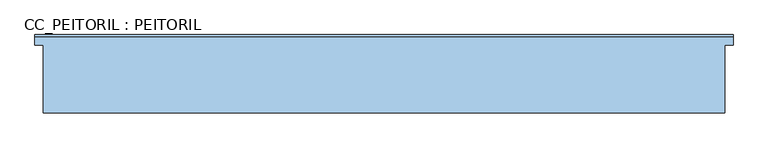
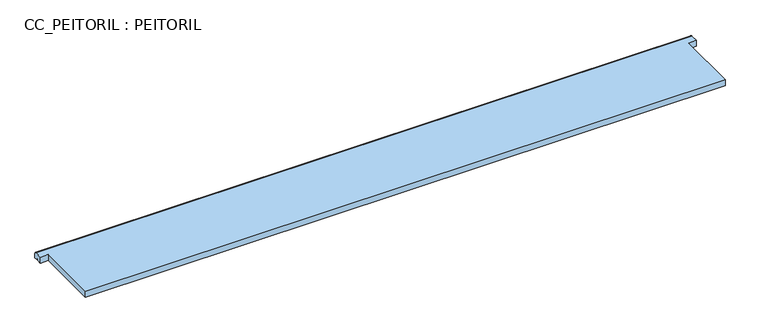
"""IFC4 building model written with IfcOpenShell, lengths in millimetres: window geometry, CC_PEITORIL : PEITORIL."""

import ifcopenshell
import ifcopenshell.guid

model = None  # the IFC model being written
_history = None  # IfcOwnerHistory: only IFC2X3 demands one
_inside = {}  # id of a spatial element -> (the spatial element, [elements in it])
_under = {}  # id of a project, library or spatial element -> (it, [spatial elements below it])
_declared = {}  # id of a project -> (the project, [libraries it declares])
_typed = {}  # id of a type object -> (the type object, [elements of that type])
_made_of = {}  # id of a material, layer set ... -> (it, [elements and type objects made of it])


def new_model(schema):
    """Start an empty IFC model of exactly this schema.

    Asked for "IFC4X3", IfcOpenShell would pick the latest addendum, in which some entities
    have other attributes; the version numbers below select the first issue.
    IFC2X3 requires an IfcOwnerHistory on every rooted entity: one is made here for all.
    """
    global model, _history
    if schema == "IFC4X3":
        model = ifcopenshell.file(schema_version=(4, 3, 0, 0))
    else:
        model = ifcopenshell.file(schema=schema)
    _inside.clear()
    _under.clear()
    _declared.clear()
    _typed.clear()
    _made_of.clear()
    _history = None
    if model.schema == "IFC2X3":
        org = make("IfcOrganization", Name="unknown")
        user = make(
            "IfcPersonAndOrganization",
            ThePerson=make("IfcPerson", FamilyName="unknown"),
            TheOrganization=org,
        )
        app = make(
            "IfcApplication",
            ApplicationDeveloper=org,
            Version="unknown",
            ApplicationFullName="unknown",
            ApplicationIdentifier="unknown",
        )
        _history = make(
            "IfcOwnerHistory",
            OwningUser=user,
            OwningApplication=app,
            ChangeAction="ADDED",
            CreationDate=0,
        )
    return model


def make(cls, **values):
    """One entity of the class cls with the attributes given. An attribute that is None is left unset."""
    return model.create_entity(
        cls, **{name: value for name, value in values.items() if value is not None}
    )


def rooted(cls, **values):
    """An entity with a GlobalId (a new one), such as an element, a storey or a relation."""
    return make(cls, GlobalId=ifcopenshell.guid.new(), OwnerHistory=_history, **values)


def si_unit(unit_type, name, prefix=None):
    """IfcSIUnit, for example si_unit("LENGTHUNIT", "METRE", prefix="MILLI")."""
    return make("IfcSIUnit", UnitType=unit_type, Prefix=prefix, Name=name)


def assignment(units):
    """IfcUnitAssignment: the units of a project."""
    return None if units is None else make("IfcUnitAssignment", Units=units)


def point(xyz):
    """IfcCartesianPoint."""
    return None if xyz is None else make("IfcCartesianPoint", Coordinates=xyz)


def direction(xyz):
    """IfcDirection."""
    return None if xyz is None else make("IfcDirection", DirectionRatios=xyz)


def frame(location, z_axis=None, x_axis=None):
    """IfcAxis2Placement3D, a coordinate frame: its origin and axes. An axis left out is left unset."""
    return make(
        "IfcAxis2Placement3D",
        Location=point(location),
        Axis=direction(z_axis),
        RefDirection=direction(x_axis),
    )


def origin():
    """The frame at (0, 0, 0) with its axes left unset."""
    return frame((0.0, 0.0, 0.0))


def place(relative_to, where):
    """IfcLocalPlacement: puts the frame where relative to a parent placement (None: the world)."""
    return make(
        "IfcLocalPlacement", PlacementRelTo=relative_to, RelativePlacement=where
    )


def context(
    kind, dimensions, precision=None, world=None, true_north=None, identifier=None
):
    """IfcGeometricRepresentationContext, for example the 3D "Model" context."""
    return make(
        "IfcGeometricRepresentationContext",
        ContextIdentifier=identifier,
        ContextType=kind,
        CoordinateSpaceDimension=dimensions,
        Precision=precision,
        WorldCoordinateSystem=world,
        TrueNorth=true_north,
    )


def project(units=None, contexts=None):
    """IfcProject with its units and contexts."""
    return rooted(
        "IfcProject",
        Name="project",
        RepresentationContexts=contexts,
        UnitsInContext=assignment(units),
    )


def spatial(cls, under=None, at=None, **own):
    """A site, building, storey or space (cls), placed at a placement, below another one or the project."""
    s = rooted(cls, ObjectPlacement=at, **own)
    if under is not None:
        _under.setdefault(under.id(), (under, []))[1].append(s)
    return s


def circle_curve(where, radius):
    """IfcCircle in the frame where."""
    return make("IfcCircle", Position=where, Radius=radius)


def shape(context_of_items, identifier, shape_type, items):
    """IfcShapeRepresentation: the items that make up one representation, for example the "Body"."""
    return make(
        "IfcShapeRepresentation",
        ContextOfItems=context_of_items,
        RepresentationIdentifier=identifier,
        RepresentationType=shape_type,
        Items=items,
    )


def source(mapping_origin, context_of_items, identifier, shape_type, items):
    """IfcRepresentationMap: a shape defined once, which mapped items show again and again."""
    return make(
        "IfcRepresentationMap",
        MappingOrigin=mapping_origin,
        MappedRepresentation=shape(context_of_items, identifier, shape_type, items),
    )


def transform(
    local_origin,
    x_axis=None,
    y_axis=None,
    z_axis=None,
    scale=None,
    scale2=None,
    scale3=None,
    uniform=True,
):
    """IfcCartesianTransformationOperator3D, or its non-uniform kind. x_axis, y_axis, z_axis: its Axis1, 2, 3."""
    if uniform:
        return make(
            "IfcCartesianTransformationOperator3D",
            Axis1=direction(x_axis),
            Axis2=direction(y_axis),
            LocalOrigin=point(local_origin),
            Scale=scale,
            Axis3=direction(z_axis),
        )
    return make(
        "IfcCartesianTransformationOperator3DnonUniform",
        Axis1=direction(x_axis),
        Axis2=direction(y_axis),
        LocalOrigin=point(local_origin),
        Scale=scale,
        Axis3=direction(z_axis),
        Scale2=scale2,
        Scale3=scale3,
    )


def mapped(mapping_source, mapping_target):
    """IfcMappedItem: shows the shape of a source again, moved by a transform."""
    return make(
        "IfcMappedItem", MappingSource=mapping_source, MappingTarget=mapping_target
    )


def made_of(thing, what):
    """Note that an element or type object is made of a material, layer set ...; save() writes the relation."""
    if what is not None:
        _made_of.setdefault(what.id(), (what, []))[1].append(thing)
    return thing


def element(
    cls,
    number,
    at=None,
    inside=None,
    cuts=None,
    type_object=None,
    material=None,
    context=None,
    identifier="Body",
    shape_type=None,
    held_by="IfcProductDefinitionShape",
    body=None,
    shapes=None,
    **own,
):
    """One element of the class cls, such as IfcWall. Its Tag is "e" and its number.

    at: its placement. inside: the storey or other place that contains it. cuts: it is an
    opening in that element (IfcRelVoidsElement). A single representation is given by context,
    identifier, shape_type and body (its items); several are given by shapes. held_by: the class
    of the entity that holds the representations. save() writes the other relations.
    """
    e = rooted(cls, Tag="e%d" % number, ObjectPlacement=at, **own)
    if body is not None:
        shapes = [shape(context, identifier, shape_type, body)]
    if shapes is not None:
        e.Representation = make(held_by, Representations=shapes)
    if inside is not None:
        _inside.setdefault(inside.id(), (inside, []))[1].append(e)
    if cuts is not None:
        rooted(
            "IfcRelVoidsElement", RelatingBuildingElement=cuts, RelatedOpeningElement=e
        )
    if type_object is not None:
        _typed.setdefault(type_object.id(), (type_object, []))[1].append(e)
    return made_of(e, material)


def aggregate(whole, parts):
    """IfcRelAggregates: a whole, such as a stair, and the parts it consists of."""
    return rooted("IfcRelAggregates", RelatingObject=whole, RelatedObjects=parts)


def save(model, path):
    """Write the relations noted so far, then the file.

    IfcRelAggregates (storeys below a building ...), IfcRelContainedInSpatialStructure (elements
    in a storey), IfcRelDefinesByType, IfcRelAssociatesMaterial and IfcRelDeclares: one each for
    every whole, place, type object, material and project.
    """
    for whole, parts in _under.values():
        aggregate(whole, parts)
    for where, things in _inside.values():
        rooted(
            "IfcRelContainedInSpatialStructure",
            RelatedElements=things,
            RelatingStructure=where,
        )
    for kind, things in _typed.values():
        rooted("IfcRelDefinesByType", RelatedObjects=things, RelatingType=kind)
    for what, things in _made_of.values():
        rooted("IfcRelAssociatesMaterial", RelatedObjects=things, RelatingMaterial=what)
    for by, libraries in _declared.values():
        rooted("IfcRelDeclares", RelatingContext=by, RelatedDefinitions=libraries)
    model.write(path)


def plane_surface(at):
    """IfcPlane: the flat surface through the origin of the frame at, square to its z axis."""
    return make("IfcPlane", Position=at)


def cylinder_surface(at, radius):
    """IfcCylindricalSurface: all points at the distance radius from the z axis of the frame at."""
    return make("IfcCylindricalSurface", Position=at, Radius=radius)


def advanced_brep(points, edges, surfaces, faces):
    """IfcAdvancedBrep: a solid bounded by faces that lie on surfaces and meet in shared edges.

    An edge is (start, end): straight between two places in points (the first is 0);
    or (start, end, curve); or (start, end, curve, False) where it runs against its curve.
    A face is (place in surfaces, loops), or (place, loops, False) where it looks against
    its surface's normal. A loop lists edges by number (the first is 1), with a minus sign
    where the edge is run from its end to its start. The first loop is the outer one.
    """
    corners = [point(p) for p in points]
    vertices = [make("IfcVertexPoint", VertexGeometry=c) for c in corners]
    made = []
    for start, end, *more in edges:
        made.append(
            make(
                "IfcEdgeCurve",
                EdgeStart=vertices[start],
                EdgeEnd=vertices[end],
                EdgeGeometry=more[0] if more else make("IfcPolyline", Points=[corners[start], corners[end]]),
                SameSense=more[1] if len(more) > 1 else True,
            )
        )
    hull = []
    for where, loops, *sense in faces:
        bounds = []
        for j, loop in enumerate(loops):
            ring = [make("IfcOrientedEdge", EdgeElement=made[abs(k) - 1], Orientation=k > 0) for k in loop]
            bounds.append(
                make(
                    "IfcFaceOuterBound" if j == 0 else "IfcFaceBound",
                    Bound=make("IfcEdgeLoop", EdgeList=ring),
                    Orientation=True,
                )
            )
        hull.append(make("IfcAdvancedFace", Bounds=bounds, FaceSurface=surfaces[where], SameSense=sense[0] if sense else True))
    return make("IfcAdvancedBrep", Outer=make("IfcClosedShell", CfsFaces=hull))


def cc_peitoril_peitoril_3c142dd7(model_context):
    return source(origin(), model_context, "Body", "AdvancedBrep", [
        advanced_brep(
        [(-1000.0, 100.0, 1500.0), (-1000.0, -100.0, 1500.0), (1000.0, -100.0, 1500.0), (1000.0, 100.0, 1500.0), (1025.0, 100.0, 1500.0), (1025.0, 123.4916648, 1500.0), (-1025.0, 123.4916648, 1500.0), (-1025.0, 100.0, 1500.0), (-1000.0, 100.0, 1480.0), (-1025.0, 100.0, 1480.0), (-1025.0, 115.0, 1480.0), (1025.0, 115.0, 1480.0), (1025.0, 100.0, 1480.0), (1000.0, 100.0, 1480.0), (1000.0, -100.0, 1480.0), (-1000.0, -100.0, 1480.0), (-1025.0, 130.0, 1480.0), (1025.0, 130.0, 1480.0), (1025.0, 120.0, 1480.0), (-1025.0, 120.0, 1480.0), (1025.0, 115.0, 1485.0), (1025.0, 120.0, 1485.0), (1025.0, 130.0, 1493.4916648), (-1025.0, 130.0, 1493.4916648), (-1025.0, 120.0, 1485.0), (-1025.0, 115.0, 1485.0)],
        [
            (0, 1),
            (1, 2),
            (2, 3),
            (3, 4),
            (4, 5),
            (5, 6),
            (6, 7),
            (7, 0),
            (8, 9),
            (9, 10),
            (10, 11),
            (11, 12),
            (12, 13),
            (13, 14),
            (14, 15),
            (15, 8),
            (16, 17),
            (17, 18),
            (18, 19),
            (19, 16),
            (0, 8),
            (15, 1),
            (14, 2),
            (13, 3),
            (12, 4),
            (11, 20),
            (20, 21),
            (21, 18),
            (17, 22),
            (22, 5, circle_curve(frame((1025.0, 123.4916648, 1493.4916648), z_axis=(1.0, 0.0, 0.0), x_axis=(0.0, -1.0, 0.0)), 6.5083352)),
            (16, 23),
            (23, 22),
            (9, 7),
            (6, 23, circle_curve(frame((-1025.0, 123.4916648, 1493.4916648), z_axis=(-1.0, 0.0, 0.0), x_axis=(0.0, -1.0, 0.0)), 6.5083352)),
            (19, 24),
            (24, 25),
            (25, 10),
            (24, 21),
            (20, 25),
        ],
        [
            plane_surface(frame((-1000.0, -100.0, 1500.0), z_axis=(0.0, 0.0, 1.0), x_axis=(0.0, -1.0, 0.0))),
            plane_surface(frame((-1000.0, -100.0, 1480.0), z_axis=(0.0, 0.0, -1.0), x_axis=(0.0, 1.0, 0.0))),
            plane_surface(frame((-1000.0, 100.0, 1500.0), z_axis=(-1.0, 0.0, 0.0), x_axis=(0.0, 0.0, -1.0))),
            plane_surface(frame((-1000.0, -100.0, 1500.0), z_axis=(0.0, -1.0, 0.0), x_axis=(0.0, 0.0, -1.0))),
            plane_surface(frame((1000.0, -100.0, 1500.0), z_axis=(1.0, 0.0, 0.0), x_axis=(0.0, 0.0, -1.0))),
            plane_surface(frame((1000.0, 100.0, 1500.0), z_axis=(0.0, -1.0, 0.0), x_axis=(0.0, 0.0, -1.0))),
            plane_surface(frame((1025.0, 100.0, 1500.0), z_axis=(1.0, 0.0, 0.0), x_axis=(0.0, 0.0, -1.0))),
            plane_surface(frame((1025.0, 130.0, 1500.0), z_axis=(0.0, 1.0, 0.0), x_axis=(0.0, 0.0, -1.0))),
            plane_surface(frame((-1025.0, 130.0, 1500.0), z_axis=(-1.0, 0.0, 0.0), x_axis=(0.0, 0.0, -1.0))),
            plane_surface(frame((-1025.0, 100.0, 1500.0), z_axis=(0.0, -1.0, 0.0), x_axis=(0.0, 0.0, -1.0))),
            cylinder_surface(frame((1025.0, 123.4916648, 1493.4916648), z_axis=(-1.0, 0.0, 0.0), x_axis=(0.0, -1.0, 0.0)), 6.5083352),
            plane_surface(frame((-1025.0, 115.0, 1485.0), z_axis=(0.0, 0.0, -1.0), x_axis=(1.0, 0.0, 0.0))),
            plane_surface(frame((-1025.0, 120.0, 1485.0), z_axis=(0.0, -1.0, 0.0), x_axis=(1.0, 0.0, 0.0))),
            plane_surface(frame((-1025.0, 115.0, 1480.0), z_axis=(0.0, 1.0, 0.0), x_axis=(1.0, 0.0, 0.0))),
        ],
        [
            (0, [[1, 2, 3, 4, 5, 6, 7, 8]]),
            (1, [[9, 10, 11, 12, 13, 14, 15, 16]]),
            (1, [[17, 18, 19, 20]]),
            (2, [[-1, 21, -16, 22]]),
            (3, [[-2, -22, -15, 23]]),
            (4, [[-3, -23, -14, 24]]),
            (5, [[-4, -24, -13, 25]]),
            (6, [[-25, -12, 26, 27, 28, -18, 29, 30, -5]]),
            (7, [[-17, 31, 32, -29]]),
            (8, [[33, -7, 34, -31, -20, 35, 36, 37, -10]]),
            (9, [[-8, -33, -9, -21]]),
            (10, [[-6, -30, -32, -34]]),
            (11, [[38, -27, 39, -36]]),
            (12, [[-38, -35, -19, -28]]),
            (13, [[-39, -26, -11, -37]]),
        ],
    ),
    ])


if __name__ == "__main__":
    model = new_model("IFC4")
    model_context = context("Model", 3, world=origin())
    ifc_project = project(units=[si_unit("LENGTHUNIT", "METRE", prefix="MILLI")], contexts=[model_context])
    site = spatial("IfcSite", under=ifc_project)
    building = spatial("IfcBuilding", under=site)
    placement = place(None, origin())
    cc_peitoril_peitoril_shape = cc_peitoril_peitoril_3c142dd7(model_context)
    element("IfcWindow", 1, ObjectType="CC_PEITORIL : PEITORIL", at=placement, inside=building, context=model_context, shape_type="MappedRepresentation", body=[
        mapped(cc_peitoril_peitoril_shape, transform((0.0, 0.0, 0.0), x_axis=(1.0, 0.0, 0.0), y_axis=(0.0, 1.0, 0.0), z_axis=(0.0, 0.0, 1.0))),
    ])
    save(model, "model.ifc")

# Revit data of these elements
# Type "CC_PEITORIL : PEITORIL"
#   Type Mark = "PEITORIL"
#   Analytic Construction = "<Nenhum>"
#   Largura da pedra [instance default] = 0.26 m
#   Interna [instance default] = 0.08 m
#   Externa [instance default] = 0.008142 m
#   Extensão Exterior [instance default] = 0.03 m
#   Extensão Exterior Esquerda [instance default] = 0.085058 m
#   Extensão Exterior Direita [instance default] = 0.10 m
#   Espessura [instance default] = 0.02 m
#   Comprimento [instance default] = 1.00 m
#   Altura-padrão do peitoril = 1.48 m
#   ----EXTENSÃO---- [instance default] = 0.00 m
#   ----DEMAIS---- [instance default] = 0.00 m
#   Peitoril [instance default] = none
#   Rough Width = 0
#   Rough Height = 0
#   Height = 0
#   Wall Closure = (empty or 0)
#   Width = 0
# Element 1 (IfcWindow, "CC_PEITORIL : PEITORIL")
#   Interna = 0.00 m
#   Externa = 0.00 m
#   Extensão Exterior Esquerda = 0.025 m
#   Extensão Exterior Direita = 0.025 m
#   Comprimento = 2.00 m
#   Peitoril = .GRANITO BRANCO ITAÚNAS
#   Materials on its faces: ".GRANITO BRANCO ITAÚNAS"
# Materials
#   ".GRANITO BRANCO ITAÚNAS": class ".CC_PEDRA REVEST.", colour RGB 202 195 174, transparency 0, Description = "Granito branco Itaúnas", Uso = "Pedra", Cost = 0
